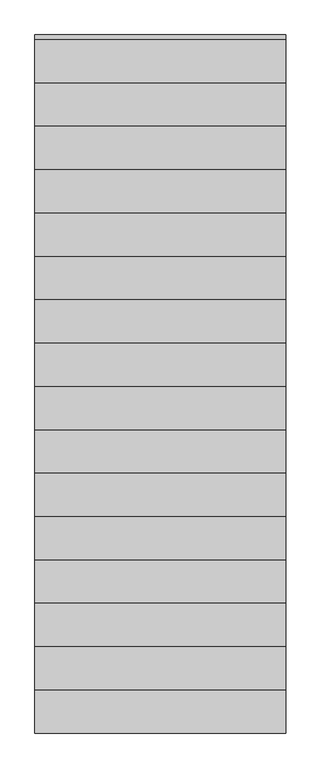
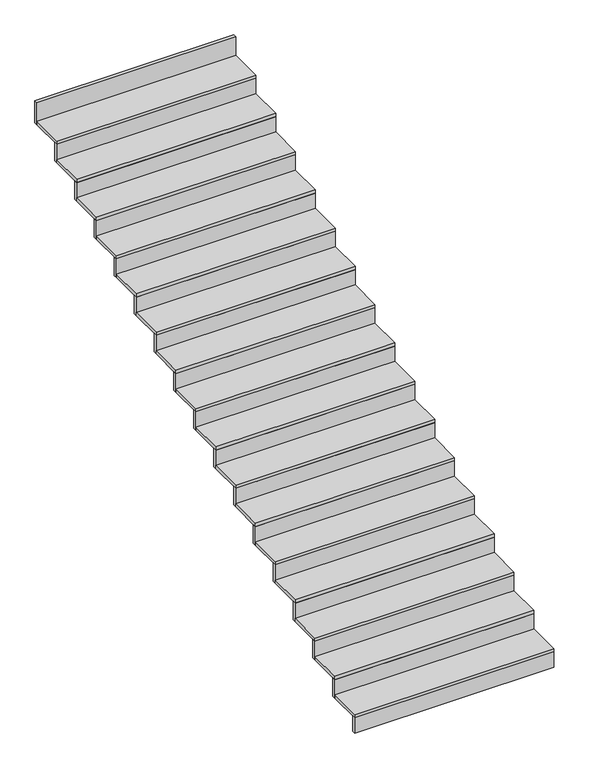
"""IFC4 building model written with IfcOpenShell, lengths in millimetres: stair flight geometry."""

from ifc_helpers import new_model, si_unit, frame, origin, place, context, project, spatial, polyline, outline, extrude, source, transform, mapped, element, save


def stair_flight_0ac641d1(model_context):
    return source(origin(), model_context, "Body", "SweptSolid", [
        extrude(outline(polyline([(52810.0, -6470.0), (52810.0, -6500.0), (51075.0, -6500.0), (51075.0, -6470.0), (52810.0, -6470.0)])), frame((0.0, 0.0, 4830.0), z_axis=(0.0, 0.0, 1.0), x_axis=(1.0, 0.0, 0.0)), (0.0, 0.0, 1.0), 140.5882353),
        extrude(outline(polyline([(51075.0, -6200.0), (52810.0, -6200.0), (52810.0, -6500.0), (51075.0, -6500.0), (51075.0, -6200.0)])), frame((0.0, 0.0, 4970.5882353), z_axis=(0.0, 0.0, 1.0), x_axis=(1.0, 0.0, 0.0)), (0.0, 0.0, 1.0), 30.0),
        extrude(outline(polyline([(52810.0, -6170.0), (52810.0, -6200.0), (51075.0, -6200.0), (51075.0, -6170.0), (52810.0, -6170.0)])), frame((0.0, 0.0, 4970.5882353), z_axis=(0.0, 0.0, 1.0), x_axis=(1.0, 0.0, 0.0)), (0.0, 0.0, 1.0), 170.5882353),
        extrude(outline(polyline([(51075.0, -5900.0), (52810.0, -5900.0), (52810.0, -6200.0), (51075.0, -6200.0), (51075.0, -5900.0)])), frame((0.0, 0.0, 5141.1764706), z_axis=(0.0, 0.0, 1.0), x_axis=(1.0, 0.0, 0.0)), (0.0, 0.0, 1.0), 30.0),
        extrude(outline(polyline([(52810.0, -5870.0), (52810.0, -5900.0), (51075.0, -5900.0), (51075.0, -5870.0), (52810.0, -5870.0)])), frame((0.0, 0.0, 5141.1764706), z_axis=(0.0, 0.0, 1.0), x_axis=(1.0, 0.0, 0.0)), (0.0, 0.0, 1.0), 170.5882353),
        extrude(outline(polyline([(51075.0, -5600.0), (52810.0, -5600.0), (52810.0, -5900.0), (51075.0, -5900.0), (51075.0, -5600.0)])), frame((0.0, 0.0, 5311.7647059), z_axis=(0.0, 0.0, 1.0), x_axis=(1.0, 0.0, 0.0)), (0.0, 0.0, 1.0), 30.0),
        extrude(outline(polyline([(52810.0, -5570.0), (52810.0, -5600.0), (51075.0, -5600.0), (51075.0, -5570.0), (52810.0, -5570.0)])), frame((0.0, 0.0, 5311.7647059), z_axis=(0.0, 0.0, 1.0), x_axis=(1.0, 0.0, 0.0)), (0.0, 0.0, 1.0), 170.5882353),
        extrude(outline(polyline([(51075.0, -5300.0), (52810.0, -5300.0), (52810.0, -5600.0), (51075.0, -5600.0), (51075.0, -5300.0)])), frame((0.0, 0.0, 5482.3529412), z_axis=(0.0, 0.0, 1.0), x_axis=(1.0, 0.0, 0.0)), (0.0, 0.0, 1.0), 30.0),
        extrude(outline(polyline([(52810.0, -5270.0), (52810.0, -5300.0), (51075.0, -5300.0), (51075.0, -5270.0), (52810.0, -5270.0)])), frame((0.0, 0.0, 5482.3529412), z_axis=(0.0, 0.0, 1.0), x_axis=(1.0, 0.0, 0.0)), (0.0, 0.0, 1.0), 170.5882353),
        extrude(outline(polyline([(51075.0, -5000.0), (52810.0, -5000.0), (52810.0, -5300.0), (51075.0, -5300.0), (51075.0, -5000.0)])), frame((0.0, 0.0, 5652.9411765), z_axis=(0.0, 0.0, 1.0), x_axis=(1.0, 0.0, 0.0)), (0.0, 0.0, 1.0), 30.0),
        extrude(outline(polyline([(52810.0, -4970.0), (52810.0, -5000.0), (51075.0, -5000.0), (51075.0, -4970.0), (52810.0, -4970.0)])), frame((0.0, 0.0, 5652.9411765), z_axis=(0.0, 0.0, 1.0), x_axis=(1.0, 0.0, 0.0)), (0.0, 0.0, 1.0), 170.5882353),
        extrude(outline(polyline([(51075.0, -4700.0), (52810.0, -4700.0), (52810.0, -5000.0), (51075.0, -5000.0), (51075.0, -4700.0)])), frame((0.0, 0.0, 5823.5294118), z_axis=(0.0, 0.0, 1.0), x_axis=(1.0, 0.0, 0.0)), (0.0, 0.0, 1.0), 30.0),
        extrude(outline(polyline([(52810.0, -4670.0), (52810.0, -4700.0), (51075.0, -4700.0), (51075.0, -4670.0), (52810.0, -4670.0)])), frame((0.0, 0.0, 5823.5294118), z_axis=(0.0, 0.0, 1.0), x_axis=(1.0, 0.0, 0.0)), (0.0, 0.0, 1.0), 170.5882353),
        extrude(outline(polyline([(51075.0, -4400.0), (52810.0, -4400.0), (52810.0, -4700.0), (51075.0, -4700.0), (51075.0, -4400.0)])), frame((0.0, 0.0, 5994.1176471), z_axis=(0.0, 0.0, 1.0), x_axis=(1.0, 0.0, 0.0)), (0.0, 0.0, 1.0), 30.0),
        extrude(outline(polyline([(52810.0, -4370.0), (52810.0, -4400.0), (51075.0, -4400.0), (51075.0, -4370.0), (52810.0, -4370.0)])), frame((0.0, 0.0, 5994.1176471), z_axis=(0.0, 0.0, 1.0), x_axis=(1.0, 0.0, 0.0)), (0.0, 0.0, 1.0), 170.5882353),
        extrude(outline(polyline([(51075.0, -4100.0), (52810.0, -4100.0), (52810.0, -4400.0), (51075.0, -4400.0), (51075.0, -4100.0)])), frame((0.0, 0.0, 6164.7058824), z_axis=(0.0, 0.0, 1.0), x_axis=(1.0, 0.0, 0.0)), (0.0, 0.0, 1.0), 30.0),
        extrude(outline(polyline([(52810.0, -4070.0), (52810.0, -4100.0), (51075.0, -4100.0), (51075.0, -4070.0), (52810.0, -4070.0)])), frame((0.0, 0.0, 6164.7058824), z_axis=(0.0, 0.0, 1.0), x_axis=(1.0, 0.0, 0.0)), (0.0, 0.0, 1.0), 170.5882353),
        extrude(outline(polyline([(51075.0, -3800.0), (52810.0, -3800.0), (52810.0, -4100.0), (51075.0, -4100.0), (51075.0, -3800.0)])), frame((0.0, 0.0, 6335.2941176), z_axis=(0.0, 0.0, 1.0), x_axis=(1.0, 0.0, 0.0)), (0.0, 0.0, 1.0), 30.0),
        extrude(outline(polyline([(52810.0, -3770.0), (52810.0, -3800.0), (51075.0, -3800.0), (51075.0, -3770.0), (52810.0, -3770.0)])), frame((0.0, 0.0, 6335.2941176), z_axis=(0.0, 0.0, 1.0), x_axis=(1.0, 0.0, 0.0)), (0.0, 0.0, 1.0), 170.5882353),
        extrude(outline(polyline([(51075.0, -3500.0), (52810.0, -3500.0), (52810.0, -3800.0), (51075.0, -3800.0), (51075.0, -3500.0)])), frame((0.0, 0.0, 6505.8823529), z_axis=(0.0, 0.0, 1.0), x_axis=(1.0, 0.0, 0.0)), (0.0, 0.0, 1.0), 30.0),
        extrude(outline(polyline([(52810.0, -3470.0), (52810.0, -3500.0), (51075.0, -3500.0), (51075.0, -3470.0), (52810.0, -3470.0)])), frame((0.0, 0.0, 6505.8823529), z_axis=(0.0, 0.0, 1.0), x_axis=(1.0, 0.0, 0.0)), (0.0, 0.0, 1.0), 170.5882353),
        extrude(outline(polyline([(51075.0, -3200.0), (52810.0, -3200.0), (52810.0, -3500.0), (51075.0, -3500.0), (51075.0, -3200.0)])), frame((0.0, 0.0, 6676.4705882), z_axis=(0.0, 0.0, 1.0), x_axis=(1.0, 0.0, 0.0)), (0.0, 0.0, 1.0), 30.0),
        extrude(outline(polyline([(52810.0, -3170.0), (52810.0, -3200.0), (51075.0, -3200.0), (51075.0, -3170.0), (52810.0, -3170.0)])), frame((0.0, 0.0, 6676.4705882), z_axis=(0.0, 0.0, 1.0), x_axis=(1.0, 0.0, 0.0)), (0.0, 0.0, 1.0), 170.5882353),
        extrude(outline(polyline([(51075.0, -2900.0), (52810.0, -2900.0), (52810.0, -3200.0), (51075.0, -3200.0), (51075.0, -2900.0)])), frame((0.0, 0.0, 6847.0588235), z_axis=(0.0, 0.0, 1.0), x_axis=(1.0, 0.0, 0.0)), (0.0, 0.0, 1.0), 30.0),
        extrude(outline(polyline([(52810.0, -2870.0), (52810.0, -2900.0), (51075.0, -2900.0), (51075.0, -2870.0), (52810.0, -2870.0)])), frame((0.0, 0.0, 6847.0588235), z_axis=(0.0, 0.0, 1.0), x_axis=(1.0, 0.0, 0.0)), (0.0, 0.0, 1.0), 170.5882353),
        extrude(outline(polyline([(51075.0, -2600.0), (52810.0, -2600.0), (52810.0, -2900.0), (51075.0, -2900.0), (51075.0, -2600.0)])), frame((0.0, 0.0, 7017.6470588), z_axis=(0.0, 0.0, 1.0), x_axis=(1.0, 0.0, 0.0)), (0.0, 0.0, 1.0), 30.0),
        extrude(outline(polyline([(52810.0, -2570.0), (52810.0, -2600.0), (51075.0, -2600.0), (51075.0, -2570.0), (52810.0, -2570.0)])), frame((0.0, 0.0, 7017.6470588), z_axis=(0.0, 0.0, 1.0), x_axis=(1.0, 0.0, 0.0)), (0.0, 0.0, 1.0), 170.5882353),
        extrude(outline(polyline([(51075.0, -2300.0), (52810.0, -2300.0), (52810.0, -2600.0), (51075.0, -2600.0), (51075.0, -2300.0)])), frame((0.0, 0.0, 7188.2352941), z_axis=(0.0, 0.0, 1.0), x_axis=(1.0, 0.0, 0.0)), (0.0, 0.0, 1.0), 30.0),
        extrude(outline(polyline([(52810.0, -2270.0), (52810.0, -2300.0), (51075.0, -2300.0), (51075.0, -2270.0), (52810.0, -2270.0)])), frame((0.0, 0.0, 7188.2352941), z_axis=(0.0, 0.0, 1.0), x_axis=(1.0, 0.0, 0.0)), (0.0, 0.0, 1.0), 170.5882353),
        extrude(outline(polyline([(51075.0, -2000.0), (52810.0, -2000.0), (52810.0, -2300.0), (51075.0, -2300.0), (51075.0, -2000.0)])), frame((0.0, 0.0, 7358.8235294), z_axis=(0.0, 0.0, 1.0), x_axis=(1.0, 0.0, 0.0)), (0.0, 0.0, 1.0), 30.0),
        extrude(outline(polyline([(52810.0, -1970.0), (52810.0, -2000.0), (51075.0, -2000.0), (51075.0, -1970.0), (52810.0, -1970.0)])), frame((0.0, 0.0, 7358.8235294), z_axis=(0.0, 0.0, 1.0), x_axis=(1.0, 0.0, 0.0)), (0.0, 0.0, 1.0), 170.5882353),
        extrude(outline(polyline([(51075.0, -1700.0), (52810.0, -1700.0), (52810.0, -2000.0), (51075.0, -2000.0), (51075.0, -1700.0)])), frame((0.0, 0.0, 7529.4117647), z_axis=(0.0, 0.0, 1.0), x_axis=(1.0, 0.0, 0.0)), (0.0, 0.0, 1.0), 30.0),
        extrude(outline(polyline([(52810.0, -1670.0), (52810.0, -1700.0), (51075.0, -1700.0), (51075.0, -1670.0), (52810.0, -1670.0)])), frame((0.0, 0.0, 7529.4117647), z_axis=(0.0, 0.0, 1.0), x_axis=(1.0, 0.0, 0.0)), (0.0, 0.0, 1.0), 200.5882353),
    ])


if __name__ == "__main__":
    model = new_model("IFC4")
    model_context = context("Model", 3, world=origin())
    ifc_project = project(units=[si_unit("LENGTHUNIT", "METRE", prefix="MILLI")], contexts=[model_context])
    site = spatial("IfcSite", under=ifc_project)
    building = spatial("IfcBuilding", under=site)
    placement = place(None, origin())
    stair_flight_shape = stair_flight_0ac641d1(model_context)
    element("IfcStairFlight", 1, at=placement, inside=building, context=model_context, shape_type="MappedRepresentation", body=[
        mapped(stair_flight_shape, transform((0.0, 0.0, 0.0), x_axis=(1.0, 0.0, 0.0), y_axis=(0.0, 1.0, 0.0), z_axis=(0.0, 0.0, 1.0))),
    ])
    save(model, "model.ifc")

# Revit data of these elements
# Element 1 (IfcStairFlight)
#   Materials on its faces: "00_Finish_Deco Tile"
# Materials
#   "00_Finish_Deco Tile": class "Finish", colour RGB 245 245 245, transparency 0, Description = "Ceramic Tile", Cost = 0
